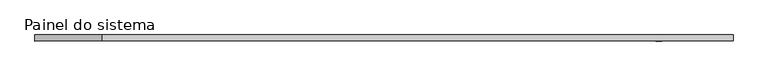
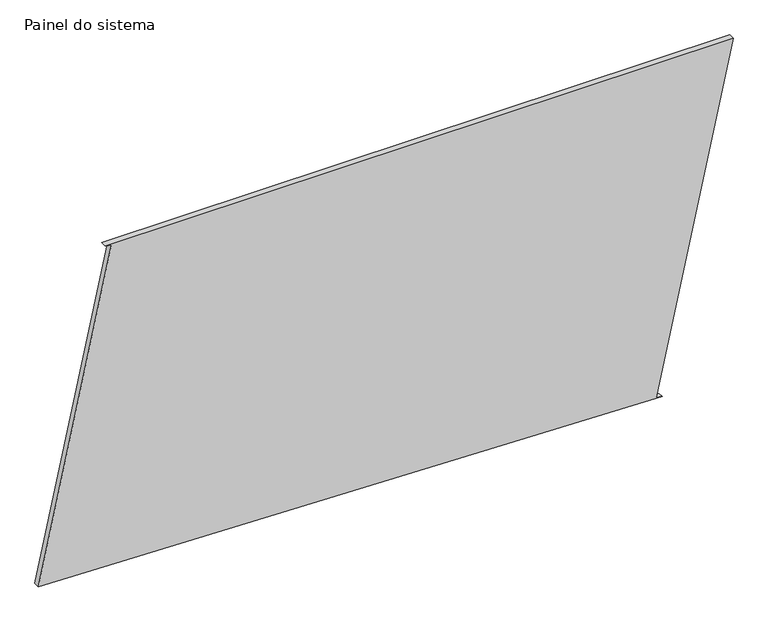
"""IFC4 building model written with IfcOpenShell, lengths in millimetres: plate geometry, Painel do sistema : Envidraçado."""

from ifc_helpers import new_model, si_unit, frame, origin, place, context, project, spatial, polyline, outline, extrude, source, transform, mapped, element, save


def painel_do_sistema_6f4e91a8(model_context):
    return source(origin(), model_context, "Body", "SweptSolid", [
        extrude(outline(polyline([(0.0, 1148.5886244), (5.3087357, 1124.1587795), (1471.9429547, 1442.8662204), (1471.9429547, -1164.2204601), (1466.6342191, -1139.7906151), (71.9348913, -1442.8662204), (0.0, 1148.5886244)])), frame((0.0, 24.5, 0.0), z_axis=(0.0, 1.0, 0.0), x_axis=(0.0, 0.0, 1.0)), (0.0, 0.0, 1.0), 25.0),
    ])


if __name__ == "__main__":
    model = new_model("IFC4")
    model_context = context("Model", 3, world=origin())
    ifc_project = project(units=[si_unit("LENGTHUNIT", "METRE", prefix="MILLI")], contexts=[model_context])
    site = spatial("IfcSite", under=ifc_project)
    building = spatial("IfcBuilding", under=site)
    placement = place(None, origin())
    painel_do_sistema_shape = painel_do_sistema_6f4e91a8(model_context)
    element("IfcPlate", 1, ObjectType="Painel do sistema : Envidraçado", at=placement, inside=building, context=model_context, shape_type="MappedRepresentation", body=[
        mapped(painel_do_sistema_shape, transform((0.0, 0.0, 0.0), x_axis=(1.0, 0.0, 0.0), y_axis=(0.0, 1.0, 0.0), z_axis=(0.0, 0.0, 1.0))),
    ])
    save(model, "model.ifc")

# Revit data of these elements
# Type "Painel do sistema : Envidraçado"
#   Construction Type Id = "GSP4R"
#   Analytic Construction = "Vidraça única Pilkington 1/8 pol"
#   Visual Light Transmittance = 0.9
#   Solar Heat Gain Coefficient = 0.86
#   Heat Transfer Coefficient (U) = 6.7069 W/(m²·K)
# Element 1 (IfcPlate, "Painel do sistema : Envidraçado")
#   Materials on its faces: "Vidro"
# Materials
#   "Vidro": class "Vidro", colour RGB 0 128 192, transparency 0.9, Description = "Vidro de sílica", Cost = 0
